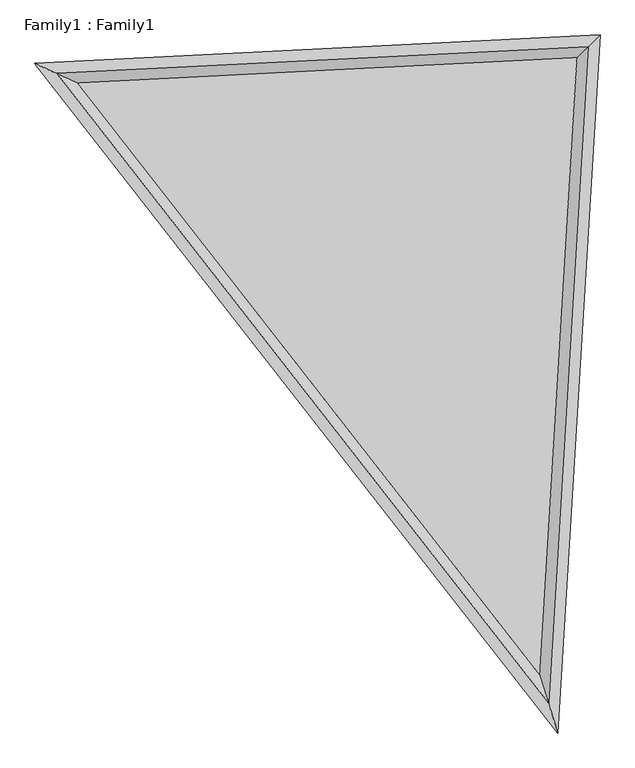
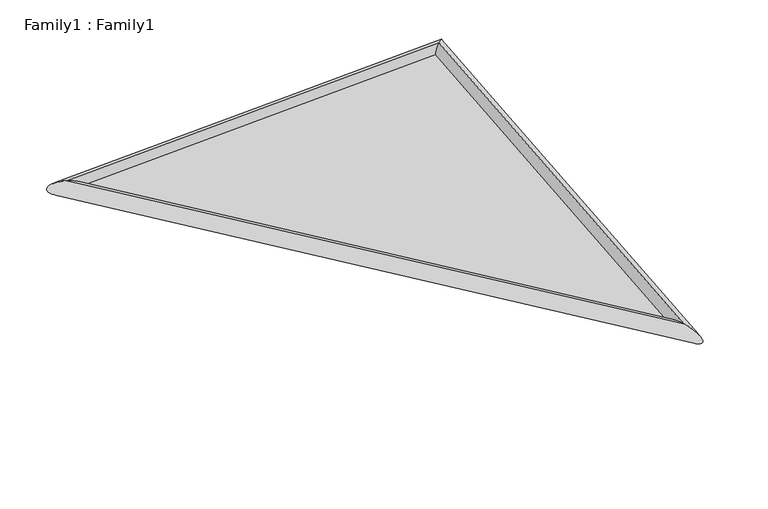
"""IFC4 building model written with IfcOpenShell, lengths in millimetres: proxy geometry, Family1 : Family1."""

from ifc_helpers import new_model, si_unit, frame, origin, origin_with_axes, place, context, project, spatial, polyline, ellipse_curve, outline, extrude, source, transform, mapped, element, save
from ifc_brep_helpers import cylinder_surface, advanced_brep


def family1_family1_6946bdc6(model_context):
    return source(origin(), model_context, "Body", "SolidModel", [
        extrude(outline(polyline([(2284.4802305, -3413.5099149), (-2160.3136544, 2277.2578236), (2642.755875, 2520.1932962), (2284.4802305, -3413.5099149)])), origin_with_axes(), (0.0, 0.0, 1.0), 34.1328789),
        advanced_brep(
        [(2284.4802305, -3413.5099149, 100.0), (2284.4802305, -3413.5099149, -100.0), (-2160.3136544, 2277.2578236, -100.0), (-2160.3136544, 2277.2578236, 100.0), (2642.755875, 2520.1932962, -100.0), (2642.755875, 2520.1932962, 100.0)],
        [
            (0, 1, ellipse_curve(frame((2284.4802305, -3413.5099149, 0.0), z_axis=(-0.9549256269430287, -0.29684515661782934, 0.0), x_axis=(0.2968451566178293, -0.9549256269430286, 0.0)), 282.598516, 100.0)),
            (1, 2),
            (2, 3, ellipse_curve(frame((-2160.3136544, 2277.2578236, 0.0), z_axis=(-0.4155884016619952, -0.9095527914332562, 0.0), x_axis=(0.909552791433256, -0.415588401661995, 0.0)), 216.918065, 100.0)),
            (3, 0),
            (1, 0, ellipse_curve(frame((2284.4802305, -3413.5099149, 0.0), z_axis=(-0.9549256269430287, -0.29684515661782934, 0.0), x_axis=(0.2968451566178293, -0.9549256269430286, 0.0)), 282.598516, 100.0)),
            (3, 2, ellipse_curve(frame((-2160.3136544, 2277.2578236, 0.0), z_axis=(-0.4155884016619952, -0.9095527914332562, 0.0), x_axis=(0.909552791433256, -0.415588401661995, 0.0)), 216.918065, 100.0)),
            (2, 4),
            (4, 5, ellipse_curve(frame((2642.755875, 2520.1932962, 0.0), z_axis=(-0.7036439960359121, 0.7105526911092612, 0.0), x_axis=(-0.7105526911092612, -0.7036439960359121, 0.0)), 149.9582316, 100.0)),
            (5, 3),
            (5, 4, ellipse_curve(frame((2642.755875, 2520.1932962, 0.0), z_axis=(-0.7036439960359121, 0.7105526911092612, 0.0), x_axis=(-0.7105526911092612, -0.7036439960359121, 0.0)), 149.9582316, 100.0)),
            (4, 1),
            (0, 5),
        ],
        [
            cylinder_surface(frame((2284.4802305, -3413.5099149, 0.0), z_axis=(0.6155478560418877, -0.7880995095305132, 0.0), x_axis=(-0.7880995095305132, -0.6155478560418877, 0.0)), 100.0),
            cylinder_surface(frame((-2160.3136544, 2277.2578236, 0.0), z_axis=(-0.9987233206835502, -0.05051463869832732, 0.0), x_axis=(-0.05051463869832732, 0.9987233206835502, 0.0)), 100.0),
            cylinder_surface(frame((2642.755875, 2520.1932962, 0.0), z_axis=(0.060270007835636914, 0.9981821107170236, 0.0), x_axis=(0.9981821107170236, -0.060270007835636914, 0.0)), 100.0),
        ],
        [
            (0, [[1, 2, 3, 4]]),
            (0, [[5, -4, 6, -2]]),
            (1, [[-3, 7, 8, 9]]),
            (1, [[-6, -9, 10, -7]]),
            (2, [[-8, 11, -1, 12]]),
            (2, [[-10, -12, -5, -11]]),
        ],
    ),
    ])


if __name__ == "__main__":
    model = new_model("IFC4")
    model_context = context("Model", 3, world=origin())
    ifc_project = project(units=[si_unit("LENGTHUNIT", "METRE", prefix="MILLI")], contexts=[model_context])
    site = spatial("IfcSite", under=ifc_project)
    building = spatial("IfcBuilding", under=site)
    placement = place(None, origin())
    family1_family1_shape = family1_family1_6946bdc6(model_context)
    element("IfcBuildingElementProxy", 1, Name="Family1 : Family1", ObjectType="Family1 : Family1", at=placement, inside=building, context=model_context, shape_type="MappedRepresentation", body=[
        mapped(family1_family1_shape, transform((0.0, 0.0, 0.0), x_axis=(1.0, 0.0, 0.0), y_axis=(0.0, 1.0, 0.0), z_axis=(0.0, 0.0, 1.0))),
    ])
    save(model, "model.ifc")

# Revit data of these elements
# Type "Family1 : Family1"
#   Default Elevation = 0
# Element 1 (IfcBuildingElementProxy, "Family1 : Family1")
#   Materials on its faces: "Glass"
# Materials
#   "Glass": class "Glass", colour RGB 0 128 192, transparency 0.9, Description = "Soda Lime Glass", Cost = 0
